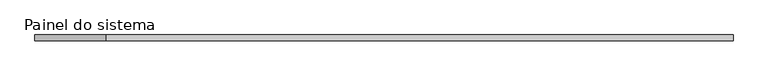
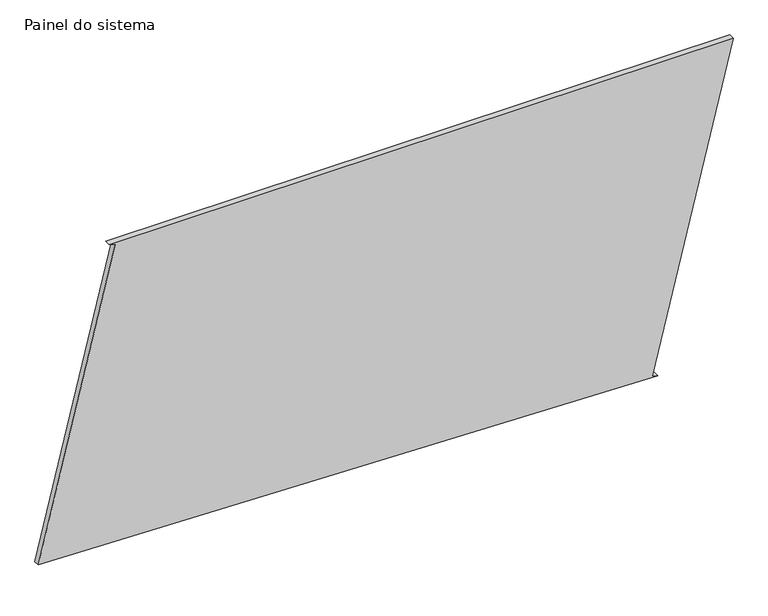
"""IFC4 building model written with IfcOpenShell, lengths in millimetres: plate geometry, Painel do sistema : Envidraçado."""

from ifc_helpers import new_model, si_unit, frame, origin, place, context, project, spatial, polyline, outline, extrude, source, transform, mapped, element, save


def painel_do_sistema_739c7000(model_context):
    return source(origin(), model_context, "Body", "SweptSolid", [
        extrude(outline(polyline([(0.0, 1144.7632755), (5.9765403, 1120.4881654), (1390.439194, 1461.3433368), (1390.439194, -1162.3614949), (1384.4626537, -1138.0863849), (71.4792665, -1461.3433368), (0.0, 1144.7632755)])), frame((0.0, 24.5, 0.0), z_axis=(0.0, 1.0, 0.0), x_axis=(0.0, 0.0, 1.0)), (0.0, 0.0, 1.0), 25.0),
    ])


if __name__ == "__main__":
    model = new_model("IFC4")
    model_context = context("Model", 3, world=origin())
    ifc_project = project(units=[si_unit("LENGTHUNIT", "METRE", prefix="MILLI")], contexts=[model_context])
    site = spatial("IfcSite", under=ifc_project)
    building = spatial("IfcBuilding", under=site)
    placement = place(None, origin())
    painel_do_sistema_shape = painel_do_sistema_739c7000(model_context)
    element("IfcPlate", 1, ObjectType="Painel do sistema : Envidraçado", at=placement, inside=building, context=model_context, shape_type="MappedRepresentation", body=[
        mapped(painel_do_sistema_shape, transform((0.0, 0.0, 0.0), x_axis=(1.0, 0.0, 0.0), y_axis=(0.0, 1.0, 0.0), z_axis=(0.0, 0.0, 1.0))),
    ])
    save(model, "model.ifc")

# Revit data of these elements
# Type "Painel do sistema : Envidraçado"
#   Construction Type Id = "GSP4R"
#   Analytic Construction = "Vidraça única Pilkington 1/8 pol"
#   Visual Light Transmittance = 0.9
#   Solar Heat Gain Coefficient = 0.86
#   Heat Transfer Coefficient (U) = 6.7069 W/(m²·K)
# Element 1 (IfcPlate, "Painel do sistema : Envidraçado")
#   Materials on its faces: "Vidro"
# Materials
#   "Vidro": class "Vidro", colour RGB 0 128 192, transparency 0.9, Description = "Vidro de sílica", Cost = 0
